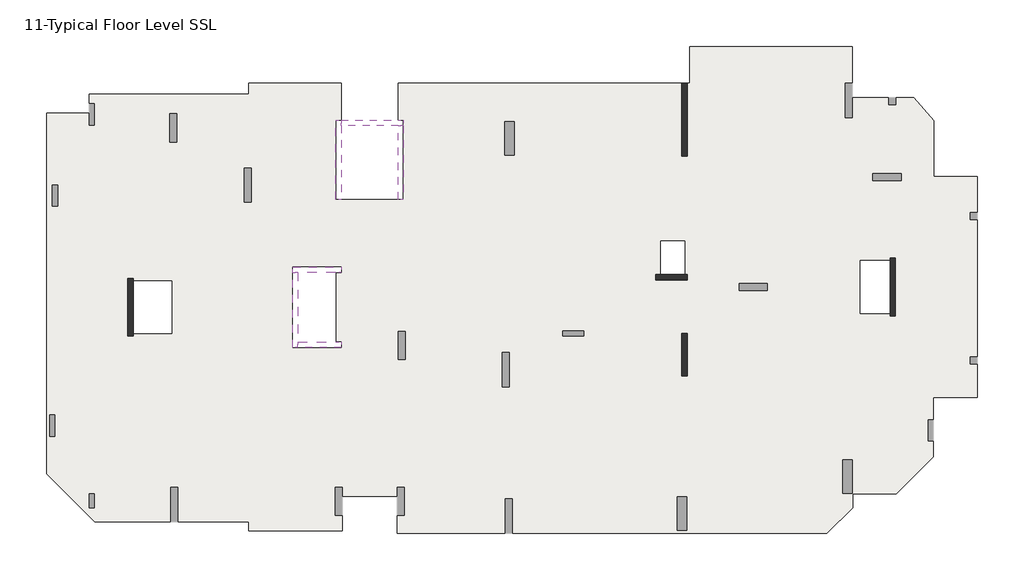
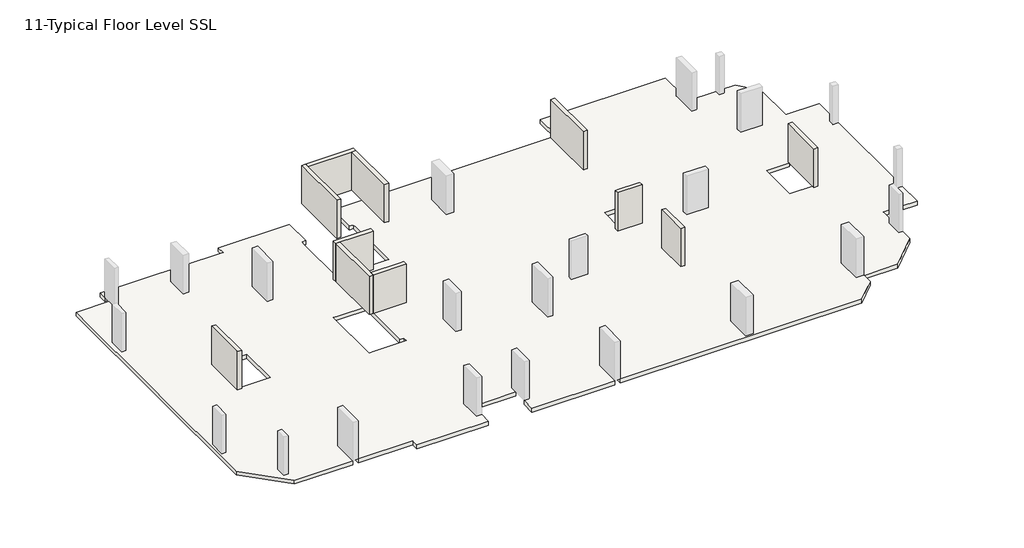
# One storey, part 1 of 2: 11 walls, 1 slab.
"""IFC4 building model written with IfcOpenShell, lengths in millimetres."""

from ifc_helpers import new_model, si_unit, origin, place, context, project, spatial, faceted_brep, element, save

model = new_model("IFC4")

# Units and contexts
model_context = context("Model", 3, world=origin())
ifc_project = project(units=[si_unit("LENGTHUNIT", "METRE", prefix="MILLI")], contexts=[model_context])

# Site, building, storey
site = spatial("IfcSite", under=ifc_project)
building = spatial("IfcBuilding", under=site)
storey = spatial("IfcBuildingStorey", under=building, Name="11-Typical Floor Level SSL", Elevation=27000.0)

# Slab
placement = place(None, origin())
element("IfcSlab", 1, ObjectType="Generic 300mm", at=placement, inside=storey, context=model_context, shape_type="Brep", body=[
    faceted_brep([(36192.0021644, 24072.000519, 26700.0), (36192.0021644, 26172.000519, 26700.0), (45446.0007483, 26172.000519, 26700.0), (45446.0007483, 24087.0, 26700.0), (45046.0007483, 24087.0, 26700.0), (45046.0007483, 22137.0, 26700.0), (45446.0007483, 22137.0, 26700.0), (45446.0007483, 23252.0000315, 26700.0), (47498.6337868, 23252.0000315, 26700.0), (47498.6337868, 22852.0, 26700.0), (47898.6337868, 22852.0, 26700.0), (47898.6337868, 23252.0000315, 26700.0), (48936.764334, 23252.0000315, 26700.0), (50076.0016214, 21956.8283806, 26700.0), (50076.0016214, 18780.0084406, 26700.0), (52549.9999998, 18780.0084406, 26700.0), (52549.9999998, 16712.0, 26700.0), (52149.9999998, 16712.0, 26700.0), (52149.9999998, 16312.0, 26700.0), (52549.9999998, 16312.0, 26700.0), (52549.9999998, 8504.0039609, 26700.0), (52149.9999998, 8504.0039609, 26700.0), (52149.9999998, 8104.0039609, 26700.0), (52549.9999998, 8104.0039609, 26700.0), (52549.9999998, 6204.0084406, 26700.0), (50046.0009271, 6204.0084406, 26700.0), (50046.0009271, 4931.9999929, 26700.0), (49746.0009271, 4931.9999929, 26700.0), (49746.0009271, 3731.9999929, 26700.0), (50046.0009271, 3731.9999929, 26700.0), (50046.0009271, 2810.5958657, 26700.0), (47943.4055804, 708.000519, 26700.0), (45456.0017287, 708.000519, 26700.0), (45456.0017287, -61.7051085, 26700.0), (43990.7023722, -1527.004465, 26700.0), (26113.9999998, -1527.004465, 26700.0), (26113.9999998, 422.995535, 26700.0), (25713.9999998, 422.995535, 26700.0), (25713.9999998, -1527.004465, 26700.0), (19569.9997488, -1527.004465, 26700.0), (19569.9997488, -512.0044652, 26700.0), (19969.9997488, -512.0044652, 26700.0), (19969.9997488, 1087.9955348, 26700.0), (19569.9997488, 1087.9955348, 26700.0), (19569.9997488, 564.000519, 26700.0), (16429.9999981, 564.000519, 26700.0), (16429.9999981, 1088.0, 26700.0), (16029.9999981, 1088.0, 26700.0), (16029.9999981, -512.0, 26700.0), (16429.9999981, -512.0, 26700.0), (16429.9999981, -1391.999481, 26700.0), (11136.0000923, -1391.999481, 26700.0), (11136.0000923, -866.9999847, 26700.0), (7082.0000416, -866.9999847, 26700.0), (7082.0000416, 1083.0000153, 26700.0), (6682.0000416, 1083.0000153, 26700.0), (6682.0000416, -866.9999847, 26700.0), (2364.4419097, -866.9999847, 26700.0), (-372.0, 1869.441925, 26700.0), (-372.0, 22380.0004589, 26700.0), (2052.0, 22380.0004589, 26700.0), (2052.0, 21708.0000656, 26700.0), (2352.0, 21708.0000656, 26700.0), (2352.0, 22908.0000656, 26700.0), (2052.0, 22908.0000656, 26700.0), (2052.0, 23472.000519, 26700.0), (11136.0000923, 23472.000519, 26700.0), (11136.0000923, 24072.000519, 26700.0), (16380.0000168, 24072.000519, 26700.0), (16380.0000168, 21972.0, 26700.0), (16079.9999997, 21972.0, 26700.0), (16079.9999997, 21672.0, 26700.0), (16079.9999997, 17468.0, 26700.0), (16379.9999997, 17468.0, 26700.0), (19619.9999997, 17468.0, 26700.0), (19919.9999997, 17468.0, 26700.0), (19919.9999997, 21672.0, 26700.0), (19919.9999997, 21972.0, 26700.0), (19619.9997365, 21972.0, 26700.0), (19619.9997365, 24072.000519, 26700.0), (35747.9999998, 24072.000519, 26700.0), (35747.9999998, 19932.0, 26700.0), (36047.9999998, 19932.0, 26700.0), (36047.9999998, 24072.000519, 26700.0), (16079.9999907, 9359.999998, 26700.0), (16079.9999907, 13320.0000002, 26700.0), (16380.0000168, 13320.0000002, 26700.0), (16380.0000168, 13620.0000002, 26700.0), (13919.9999907, 13620.0000002, 26700.0), (13619.9999907, 13620.0000002, 26700.0), (13619.9999907, 13320.0000002, 26700.0), (13619.9999907, 9359.999998, 26700.0), (13619.9999907, 9059.999998, 26700.0), (13919.9999907, 9059.999998, 26700.0), (16380.0000168, 9059.999998, 26700.0), (16380.0000168, 9359.999998, 26700.0), (4548.0000034, 9840.0000003, 26700.0), (6743.9999995, 9840.0000003, 26700.0), (6743.9999995, 12840.0000003, 26700.0), (4548.0000034, 12840.0000003, 26700.0), (4548.0000025, 12984.0000001, 26700.0), (4248.0000025, 12984.0000001, 26700.0), (4248.0000025, 9696.0, 26700.0), (4548.0000025, 9696.0, 26700.0), (47580.0014798, 13992.0079177, 26700.0), (45900.001729, 13992.0079177, 26700.0), (45900.001729, 10992.0079181, 26700.0), (47580.0014798, 10992.0079181, 26700.0), (47580.0014811, 10848.0079202, 26700.0), (47880.0014811, 10848.0079202, 26700.0), (47880.0014811, 14136.0000002, 26700.0), (47580.0014811, 14136.0000002, 26700.0), (35904.002157, 15108.0000083, 26700.0), (34548.0015145, 15108.0000083, 26700.0), (34548.0015145, 13199.9999992, 26700.0), (34248.0015201, 13199.9999992, 26700.0), (34248.0015201, 12899.9999992, 26700.0), (36048.0015201, 12899.9999992, 26700.0), (36048.0015201, 13199.9999992, 26700.0), (35904.002157, 13199.9999992, 26700.0), (257.9999999, 17088.0, 26700.0), (257.9999999, 18288.0, 26700.0), (-42.0000001, 18288.0, 26700.0), (-42.0000001, 17088.0, 26700.0), (108.001803, 4001.9999858, 26700.0), (108.001803, 5201.9999858, 26700.0), (-191.998197, 5201.9999858, 26700.0), (-191.998197, 4001.9999858, 26700.0), (30175.9999998, 9996.0000019, 26700.0), (28975.9999998, 9996.0000019, 26700.0), (28975.9999998, 9696.0000019, 26700.0), (30175.9999998, 9696.0000019, 26700.0), (7021.9999999, 20740.0000078, 26700.0), (7021.9999999, 22340.0000078, 26700.0), (6621.9999999, 22340.0000078, 26700.0), (6621.9999999, 20740.0000078, 26700.0), (48205.9993605, 18950.0, 26700.0), (46605.9993605, 18950.0, 26700.0), (46605.9993605, 18550.0, 26700.0), (48205.9993605, 18550.0, 26700.0), (20030.000009, 8355.9999979, 26700.0), (20030.000009, 9955.9999979, 26700.0), (19630.000009, 9955.9999979, 26700.0), (19630.000009, 8355.9999979, 26700.0), (11270.0000427, 17312.9999996, 26700.0), (11270.0000427, 19262.9999996, 26700.0), (10870.0000427, 19262.9999996, 26700.0), (10870.0000427, 17312.9999996, 26700.0), (40598.0014887, 12692.0079212, 26700.0), (38998.0014887, 12692.0079212, 26700.0), (38998.0014887, 12292.0079212, 26700.0), (40598.0014887, 12292.0079212, 26700.0), (2352.0, -72.0, 26700.0), (2352.0, 728.0, 26700.0), (2052.0, 728.0, 26700.0), (2052.0, -72.0, 26700.0), (25934.0000455, 6801.0001824, 26700.0), (25934.0000455, 8751.0001824, 26700.0), (25534.0000455, 8751.0001824, 26700.0), (25534.0000455, 6801.0001824, 26700.0), (36035.9999998, -1351.9992017, 26700.0), (36035.9999998, 548.0007983, 26700.0), (35485.9999998, 548.0007983, 26700.0), (35485.9999998, -1351.9992017, 26700.0), (45443.9999998, 748.0, 26700.0), (45443.9999998, 2648.0, 26700.0), (44893.9999998, 2648.0, 26700.0), (44893.9999998, 748.0, 26700.0), (26218.9999998, 20000.0, 26700.0), (26218.9999998, 21900.0, 26700.0), (25668.9999998, 21900.0, 26700.0), (25668.9999998, 20000.0, 26700.0), (35748.0054035, 9840.0000002, 26700.0), (35748.0054035, 7428.0000762, 26700.0), (36048.0054035, 7428.0000762, 26700.0), (36048.0054035, 9840.0000002, 26700.0), (36192.0021644, 26172.000519, 27000.0), (36192.0021644, 24072.000519, 27000.0), (36047.9999998, 24072.000519, 27000.0), (36047.9999998, 19932.0, 27000.0), (35747.9999998, 19932.0, 27000.0), (35747.9999998, 24072.000519, 27000.0), (19619.9997365, 24072.000519, 27000.0), (19619.9997365, 21972.0, 27000.0), (19919.9999997, 21972.0, 27000.0), (19919.9999997, 21672.0, 27000.0), (19919.9999997, 17468.0, 27000.0), (19619.9999997, 17468.0, 27000.0), (16379.9999997, 17468.0, 27000.0), (16079.9999997, 17468.0, 27000.0), (16079.9999997, 21672.0, 27000.0), (16079.9999997, 21972.0, 27000.0), (16380.0000168, 21972.0, 27000.0), (16380.0000168, 24072.000519, 27000.0), (11136.0000923, 24072.000519, 27000.0), (11136.0000923, 23472.000519, 27000.0), (2052.0, 23472.000519, 27000.0), (2052.0, 22908.0000656, 27000.0), (2352.0, 22908.0000656, 27000.0), (2352.0, 21708.0000656, 27000.0), (2052.0, 21708.0000656, 27000.0), (2052.0, 22380.0004589, 27000.0), (-372.0, 22380.0004589, 27000.0), (-372.0, 1869.441925, 27000.0), (2364.4419097, -866.9999847, 27000.0), (6682.0000416, -866.9999847, 27000.0), (6682.0000416, 1083.0000153, 27000.0), (7082.0000416, 1083.0000153, 27000.0), (7082.0000416, -866.9999847, 27000.0), (11136.0000923, -866.9999847, 27000.0), (11136.0000923, -1391.999481, 27000.0), (16429.9999981, -1391.999481, 27000.0), (16429.9999981, -512.0, 27000.0), (16029.9999981, -512.0, 27000.0), (16029.9999981, 1088.0, 27000.0), (16429.9999981, 1088.0, 27000.0), (16429.9999981, 564.000519, 27000.0), (19569.9997488, 564.000519, 27000.0), (19569.9997488, 1087.9955348, 27000.0), (19969.9997488, 1087.9955348, 27000.0), (19969.9997488, -512.0044652, 27000.0), (19569.9997488, -512.0044652, 27000.0), (19569.9997488, -1527.004465, 27000.0), (25713.9999998, -1527.004465, 27000.0), (25713.9999998, 422.995535, 27000.0), (26113.9999998, 422.995535, 27000.0), (26113.9999998, -1527.004465, 27000.0), (43990.7023722, -1527.004465, 27000.0), (45456.0017287, -61.7051085, 27000.0), (45456.0017287, 708.000519, 27000.0), (47943.4055804, 708.000519, 27000.0), (50046.0009271, 2810.5958657, 27000.0), (50046.0009271, 3731.9999929, 27000.0), (49746.0009271, 3731.9999929, 27000.0), (49746.0009271, 4931.9999929, 27000.0), (50046.0009271, 4931.9999929, 27000.0), (50046.0009271, 6204.0084406, 27000.0), (52549.9999998, 6204.0084406, 27000.0), (52549.9999998, 8104.0039609, 27000.0), (52149.9999998, 8104.0039609, 27000.0), (52149.9999998, 8504.0039609, 27000.0), (52549.9999998, 8504.0039609, 27000.0), (52549.9999998, 16312.0, 27000.0), (52149.9999998, 16312.0, 27000.0), (52149.9999998, 16712.0, 27000.0), (52549.9999998, 16712.0, 27000.0), (52549.9999998, 18780.0084406, 27000.0), (50076.0016214, 18780.0084406, 27000.0), (50076.0016214, 21956.8283806, 27000.0), (48936.764334, 23252.0000315, 27000.0), (47898.6337868, 23252.0000315, 27000.0), (47898.6337868, 22852.0, 27000.0), (47498.6337868, 22852.0, 27000.0), (47498.6337868, 23252.0000315, 27000.0), (45446.0006898, 23252.0000315, 27000.0), (45446.0007483, 22137.0, 27000.0), (45046.0007483, 22137.0, 27000.0), (45046.0007483, 24087.0, 27000.0), (45446.0007483, 24087.0, 27000.0), (45446.0007483, 26172.000519, 27000.0), (16079.9999907, 13320.0000002, 27000.0), (16079.9999907, 9359.999998, 27000.0), (16380.0000168, 9359.999998, 27000.0), (16380.0000168, 9059.999998, 27000.0), (13919.9999907, 9059.999998, 27000.0), (13619.9999907, 9059.999998, 27000.0), (13619.9999907, 9359.999998, 27000.0), (13619.9999907, 13320.0000002, 27000.0), (13619.9999907, 13620.0000002, 27000.0), (13919.9999907, 13620.0000002, 27000.0), (16380.0000168, 13620.0000002, 27000.0), (16380.0000168, 13320.0000002, 27000.0), (6743.9999995, 9840.0000003, 27000.0), (4548.0000034, 9840.0000003, 27000.0), (4548.0000025, 9696.0, 27000.0), (4248.0000025, 9696.0, 27000.0), (4248.0000025, 12984.0000001, 27000.0), (4548.0000025, 12984.0000001, 27000.0), (4548.0000025, 12840.0000003, 27000.0), (6743.9999995, 12840.0000003, 27000.0), (45900.001729, 13992.0079177, 27000.0), (47580.0014798, 13992.0079177, 27000.0), (47580.0014811, 14136.0000002, 27000.0), (47880.0014811, 14136.0000002, 27000.0), (47880.0014811, 10848.0079202, 27000.0), (47580.0014811, 10848.0079202, 27000.0), (47580.0014811, 10992.0079181, 27000.0), (45900.001729, 10992.0079181, 27000.0), (34548.0015145, 15108.0000083, 27000.0), (35904.002157, 15108.0000083, 27000.0), (35904.002157, 13199.9999992, 27000.0), (36048.0015201, 13199.9999992, 27000.0), (36048.0015201, 12899.9999992, 27000.0), (34248.0015201, 12899.9999992, 27000.0), (34248.0015201, 13199.9999992, 27000.0), (34548.0015145, 13199.9999992, 27000.0), (257.9999999, 18288.0, 27000.0), (257.9999999, 17088.0, 27000.0), (-42.0000001, 17088.0, 27000.0), (-42.0000001, 18288.0, 27000.0), (108.001803, 5201.9999858, 27000.0), (108.001803, 4001.9999858, 27000.0), (-191.998197, 4001.9999858, 27000.0), (-191.998197, 5201.9999858, 27000.0), (28975.9999998, 9996.0000019, 27000.0), (30175.9999998, 9996.0000019, 27000.0), (30175.9999998, 9696.0000019, 27000.0), (28975.9999998, 9696.0000019, 27000.0), (7021.9999999, 22340.0000078, 27000.0), (7021.9999999, 20740.0000078, 27000.0), (6621.9999999, 20740.0000078, 27000.0), (6621.9999999, 22340.0000078, 27000.0), (46605.9993605, 18950.0, 27000.0), (48205.9993605, 18950.0, 27000.0), (48205.9993605, 18550.0, 27000.0), (46605.9993605, 18550.0, 27000.0), (20030.000009, 9955.9999979, 27000.0), (20030.000009, 8355.9999979, 27000.0), (19630.000009, 8355.9999979, 27000.0), (19630.000009, 9955.9999979, 27000.0), (11270.0000427, 19262.9999996, 27000.0), (11270.0000427, 17312.9999996, 27000.0), (10870.0000427, 17312.9999996, 27000.0), (10870.0000427, 19262.9999996, 27000.0), (38998.0014887, 12692.0079212, 27000.0), (40598.0014887, 12692.0079212, 27000.0), (40598.0014887, 12292.0079212, 27000.0), (38998.0014887, 12292.0079212, 27000.0), (2352.0, 728.0, 27000.0), (2352.0, -72.0, 27000.0), (2052.0, -72.0, 27000.0), (2052.0, 728.0, 27000.0), (25934.0000455, 8751.0001824, 27000.0), (25934.0000455, 6801.0001824, 27000.0), (25534.0000455, 6801.0001824, 27000.0), (25534.0000455, 8751.0001824, 27000.0), (36035.9999998, 548.0007983, 27000.0), (36035.9999998, -1351.9992017, 27000.0), (35485.9999998, -1351.9992017, 27000.0), (35485.9999998, 548.0007983, 27000.0), (45443.9999998, 2648.0, 27000.0), (45443.9999998, 748.0, 27000.0), (44893.9999998, 748.0, 27000.0), (44893.9999998, 2648.0, 27000.0), (26218.9999998, 21900.0, 27000.0), (26218.9999998, 20000.0, 27000.0), (25668.9999998, 20000.0, 27000.0), (25668.9999998, 21900.0, 27000.0), (35748.0054035, 7428.0000762, 27000.0), (35748.0054035, 9840.0000002, 27000.0), (36048.0054035, 9840.0000002, 27000.0), (36048.0054035, 7428.0000762, 27000.0)], [[[0, 1, 2, 3, 4, 5, 6, 7, 8, 9, 10, 11, 12, 13, 14, 15, 16, 17, 18, 19, 20, 21, 22, 23, 24, 25, 26, 27, 28, 29, 30, 31, 32, 33, 34, 35, 36, 37, 38, 39, 40, 41, 42, 43, 44, 45, 46, 47, 48, 49, 50, 51, 52, 53, 54, 55, 56, 57, 58, 59, 60, 61, 62, 63, 64, 65, 66, 67, 68, 69, 70, 71, 72, 73, 74, 75, 76, 77, 78, 79, 80, 81, 82, 83], [84, 85, 86, 87, 88, 89, 90, 91, 92, 93, 94, 95], [96, 97, 98, 99, 100, 101, 102, 103], [104, 105, 106, 107, 108, 109, 110, 111], [112, 113, 114, 115, 116, 117, 118, 119], [120, 121, 122, 123], [124, 125, 126, 127], [128, 129, 130, 131], [132, 133, 134, 135], [136, 137, 138, 139], [140, 141, 142, 143], [144, 145, 146, 147], [148, 149, 150, 151], [152, 153, 154, 155], [156, 157, 158, 159], [160, 161, 162, 163], [164, 165, 166, 167], [168, 169, 170, 171], [172, 173, 174, 175]], [[176, 177, 178, 179, 180, 181, 182, 183, 184, 185, 186, 187, 188, 189, 190, 191, 192, 193, 194, 195, 196, 197, 198, 199, 200, 201, 202, 203, 204, 205, 206, 207, 208, 209, 210, 211, 212, 213, 214, 215, 216, 217, 218, 219, 220, 221, 222, 223, 224, 225, 226, 227, 228, 229, 230, 231, 232, 233, 234, 235, 236, 237, 238, 239, 240, 241, 242, 243, 244, 245, 246, 247, 248, 249, 250, 251, 252, 253, 254, 255, 256, 257, 258, 259], [260, 261, 262, 263, 264, 265, 266, 267, 268, 269, 270, 271], [272, 273, 274, 275, 276, 277, 278, 279], [280, 281, 282, 283, 284, 285, 286, 287], [288, 289, 290, 291, 292, 293, 294, 295], [296, 297, 298, 299], [300, 301, 302, 303], [304, 305, 306, 307], [308, 309, 310, 311], [312, 313, 314, 315], [316, 317, 318, 319], [320, 321, 322, 323], [324, 325, 326, 327], [328, 329, 330, 331], [332, 333, 334, 335], [336, 337, 338, 339], [340, 341, 342, 343], [344, 345, 346, 347], [348, 349, 350, 351]], [[68, 193, 192, 69]], [[182, 79, 78, 183]], [[79, 182, 181, 80]], [[177, 0, 83, 178]], [[1, 0, 177, 176]], [[2, 1, 176, 259]], [[3, 2, 259, 258]], [[249, 12, 11, 250]], [[7, 254, 253, 8]], [[13, 12, 249, 248]], [[14, 13, 248, 247]], [[15, 14, 247, 246]], [[15, 246, 245, 16]], [[237, 24, 23, 238]], [[19, 242, 241, 20]], [[25, 24, 237, 236]], [[25, 236, 235, 26]], [[231, 30, 29, 232]], [[32, 31, 230, 229]], [[33, 32, 229, 228]], [[34, 33, 228, 227]], [[34, 227, 226, 35]], [[222, 39, 38, 223]], [[39, 222, 221, 40]], [[45, 44, 217, 216]], [[211, 50, 49, 212]], [[51, 50, 211, 210]], [[52, 51, 210, 209]], [[52, 209, 208, 53]], [[204, 57, 56, 205]], [[58, 57, 204, 203]], [[59, 58, 203, 202]], [[60, 59, 202, 201]], [[196, 65, 64, 197]], [[66, 65, 196, 195]], [[67, 66, 195, 194]], [[68, 67, 194, 193]], [[31, 30, 231, 230]], [[85, 84, 261, 260]], [[72, 189, 188, 187, 186, 75, 74, 73]], [[272, 97, 96, 273]], [[97, 272, 279, 98]], [[98, 279, 278, 99]], [[280, 105, 104, 281]], [[105, 280, 287, 106]], [[106, 287, 286, 107]], [[112, 289, 288, 113]], [[113, 288, 295, 114]], [[289, 112, 119, 290]], [[62, 199, 198, 63]], [[199, 62, 61, 200]], [[200, 61, 60, 201]], [[63, 198, 197, 64]], [[120, 297, 296, 121]], [[297, 120, 123, 298]], [[298, 123, 122, 299]], [[299, 122, 121, 296]], [[124, 301, 300, 125]], [[301, 124, 127, 302]], [[302, 127, 126, 303]], [[303, 126, 125, 300]], [[28, 233, 232, 29]], [[233, 28, 27, 234]], [[234, 27, 26, 235]], [[128, 305, 304, 129]], [[305, 128, 131, 306]], [[306, 131, 130, 307]], [[307, 130, 129, 304]], [[132, 309, 308, 133]], [[309, 132, 135, 310]], [[310, 135, 134, 311]], [[311, 134, 133, 308]], [[41, 220, 219, 42]], [[220, 41, 40, 221]], [[43, 218, 217, 44]], [[218, 43, 42, 219]], [[136, 313, 312, 137]], [[313, 136, 139, 314]], [[314, 139, 138, 315]], [[315, 138, 137, 312]], [[140, 317, 316, 141]], [[317, 140, 143, 318]], [[318, 143, 142, 319]], [[319, 142, 141, 316]], [[215, 46, 45, 216]], [[48, 213, 212, 49]], [[213, 48, 47, 214]], [[214, 47, 46, 215]], [[144, 321, 320, 145]], [[321, 144, 147, 322]], [[322, 147, 146, 323]], [[323, 146, 145, 320]], [[207, 54, 53, 208]], [[55, 206, 205, 56]], [[206, 55, 54, 207]], [[225, 36, 35, 226]], [[37, 224, 223, 38]], [[224, 37, 36, 225]], [[6, 255, 254, 7]], [[255, 6, 5, 256]], [[256, 5, 4, 257]], [[257, 4, 3, 258]], [[148, 325, 324, 149]], [[325, 148, 151, 326]], [[326, 151, 150, 327]], [[327, 150, 149, 324]], [[152, 329, 328, 153]], [[329, 152, 155, 330]], [[330, 155, 154, 331]], [[331, 154, 153, 328]], [[156, 333, 332, 157]], [[333, 156, 159, 334]], [[334, 159, 158, 335]], [[335, 158, 157, 332]], [[160, 337, 336, 161]], [[337, 160, 163, 338]], [[338, 163, 162, 339]], [[339, 162, 161, 336]], [[164, 341, 340, 165]], [[341, 164, 167, 342]], [[342, 167, 166, 343]], [[343, 166, 165, 340]], [[168, 345, 344, 169]], [[345, 168, 171, 346]], [[346, 171, 170, 347]], [[347, 170, 169, 344]], [[70, 191, 190, 189, 72, 71]], [[191, 70, 69, 192]], [[77, 184, 183, 78]], [[184, 77, 76, 75, 186, 185]], [[271, 86, 85, 260]], [[87, 270, 269, 268, 89, 88]], [[86, 271, 270, 87]], [[89, 268, 267, 266, 265, 92, 91, 90]], [[92, 265, 264, 263, 94, 93]], [[95, 262, 261, 84]], [[262, 95, 94, 263]], [[277, 100, 99, 278]], [[103, 274, 273, 96]], [[101, 276, 275, 102]], [[100, 277, 276, 101]], [[274, 103, 102, 275]], [[116, 293, 292, 117]], [[118, 291, 290, 119]], [[294, 115, 114, 295]], [[117, 292, 291, 118]], [[293, 116, 115, 294]], [[172, 349, 348, 173]], [[174, 351, 350, 175]], [[173, 348, 351, 174]], [[349, 172, 175, 350]], [[285, 108, 107, 286]], [[111, 282, 281, 104]], [[109, 284, 283, 110]], [[108, 285, 284, 109]], [[282, 111, 110, 283]], [[82, 179, 178, 83]], [[180, 81, 80, 181]], [[179, 82, 81, 180]], [[18, 243, 242, 19]], [[243, 18, 17, 244]], [[244, 17, 16, 245]], [[10, 251, 250, 11]], [[251, 10, 9, 252]], [[252, 9, 8, 253]], [[22, 239, 238, 23]], [[239, 22, 21, 240]], [[240, 21, 20, 241]]]),
])

# Walls
element("IfcWall", 2, ObjectType="Shear Walls 300mm", at=placement, inside=storey, context=model_context, shape_type="Brep", body=[
    faceted_brep([(4548.0000025, 9696.0, 27000.0), (4548.0000025, 12984.0000001, 27000.0), (4548.0000025, 12984.0000001, 29700.0), (4548.0000025, 12984.0000001, 30000.0), (4548.0000025, 12840.0000003, 30000.0), (4548.0000025, 9840.0000003, 30000.0), (4548.0000025, 9696.0, 30000.0), (4548.0000025, 9696.0, 29700.0), (4248.0000025, 9696.0, 27000.0), (4248.0000025, 9696.0, 29700.0), (4248.0000025, 9696.0, 30000.0), (4248.0000025, 12984.0000001, 30000.0), (4248.0000025, 12984.0000001, 29700.0), (4248.0000025, 12984.0000001, 27000.0)], [[[0, 1, 2, 3, 4, 5, 6, 7]], [[8, 9, 10, 11, 12, 13]], [[1, 0, 8, 13]], [[3, 2, 1, 13, 12, 11]], [[6, 5, 4, 3, 11, 10]], [[0, 7, 6, 10, 9, 8]]]),
])
element("IfcWall", 3, ObjectType="Shear Walls 300mm", at=placement, inside=storey, context=model_context, shape_type="Brep", body=[
    faceted_brep([(34248.0015201, 12899.9999992, 27000.0), (36048.0015201, 12899.9999992, 27000.0), (36048.0015201, 12899.9999992, 29700.0), (36048.0015201, 12899.9999992, 30000.0), (34248.0015201, 12899.9999992, 30000.0), (34248.0015201, 12899.9999992, 29700.0), (34248.0015201, 13199.9999992, 27000.0), (34248.0015201, 13199.9999992, 29700.0), (34248.0015201, 13199.9999992, 30000.0), (34548.0015145, 13199.9999992, 30000.0), (35904.002157, 13199.9999992, 30000.0), (36048.0015201, 13199.9999992, 30000.0), (36048.0015201, 13199.9999992, 29700.0), (36048.0015201, 13199.9999992, 27000.0)], [[[0, 1, 2, 3, 4, 5]], [[6, 7, 8, 9, 10, 11, 12, 13]], [[1, 0, 6, 13]], [[3, 2, 1, 13, 12, 11]], [[4, 3, 11, 10, 9, 8]], [[0, 5, 4, 8, 7, 6]]]),
])
element("IfcWall", 4, ObjectType="Shear Walls 300mm", at=placement, inside=storey, context=model_context, shape_type="Brep", body=[
    faceted_brep([(35748.0054035, 9840.0000002, 27000.0), (35748.0054035, 7428.0000762, 27000.0), (35748.0054035, 7428.0000762, 29700.0), (35748.0054035, 7428.0000762, 30000.0), (35748.0054035, 9840.0000002, 30000.0), (35748.0054035, 9840.0000002, 29700.0), (36048.0054035, 9840.0000002, 27000.0), (36048.0054035, 9840.0000002, 29700.0), (36048.0054035, 9840.0000002, 30000.0), (36048.0054035, 7428.0000762, 30000.0), (36048.0054035, 7428.0000762, 29700.0), (36048.0054035, 7428.0000762, 27000.0)], [[[0, 1, 2, 3, 4, 5]], [[6, 7, 8, 9, 10, 11]], [[1, 0, 6, 11]], [[3, 2, 1, 11, 10, 9]], [[4, 3, 9, 8]], [[0, 5, 4, 8, 7, 6]]]),
])
element("IfcWall", 5, ObjectType="Shear Walls 300mm", at=placement, inside=storey, context=model_context, shape_type="Brep", body=[
    faceted_brep([(47580.0014811, 14136.0000002, 27000.0), (47580.0014811, 10848.0079202, 27000.0), (47580.0014811, 10848.0079202, 29700.0), (47580.0014811, 10848.0079202, 30000.0), (47580.0014811, 10992.0079181, 30000.0), (47580.0014811, 13992.0079177, 30000.0), (47580.0014811, 14136.0000002, 30000.0), (47580.0014811, 14136.0000002, 29700.0), (47880.0014811, 14136.0000002, 27000.0), (47880.0014811, 14136.0000002, 29700.0), (47880.0014811, 14136.0000002, 30000.0), (47880.0014811, 10848.0079202, 30000.0), (47880.0014811, 10848.0079202, 29700.0), (47880.0014811, 10848.0079202, 27000.0)], [[[0, 1, 2, 3, 4, 5, 6, 7]], [[8, 9, 10, 11, 12, 13]], [[1, 0, 8, 13]], [[3, 2, 1, 13, 12, 11]], [[6, 5, 4, 3, 11, 10]], [[0, 7, 6, 10, 9, 8]]]),
])
element("IfcWall", 6, ObjectType="Shear Walls 300mm", at=placement, inside=storey, context=model_context, shape_type="Brep", body=[
    faceted_brep([(36047.9999998, 19932.0, 27000.0), (36047.9999998, 24072.0078999, 27000.0), (36047.9999998, 24072.0078999, 30000.0), (36047.9999998, 19932.0, 30000.0), (36047.9999998, 19932.0, 29700.0), (35747.9999998, 19932.0, 27000.0), (35747.9999998, 19932.0, 29700.0), (35747.9999998, 19932.0, 30000.0), (35747.9999998, 24072.0078999, 30000.0), (35747.9999998, 24072.0078999, 27000.0)], [[[0, 1, 2, 3, 4]], [[5, 6, 7, 8, 9]], [[1, 0, 5, 9]], [[2, 1, 9, 8]], [[3, 2, 8, 7]], [[0, 4, 3, 7, 6, 5]]]),
])
element("IfcWall", 7, ObjectType="Shear Walls 300mm", at=placement, inside=storey, context=model_context, shape_type="Brep", body=[
    faceted_brep([(16379.9999997, 21972.0, 33000.0), (16379.9999997, 21672.0, 33000.0), (16379.9999997, 17468.0, 33000.0), (16379.9999997, 17468.0, 30000.0), (16379.9999997, 21672.0, 30000.0), (16379.9999997, 21972.0, 30000.0), (16079.9999997, 17468.0, 33000.0), (16079.9999997, 21972.0, 33000.0), (16079.9999997, 21972.0, 32700.0), (16079.9999997, 21972.0, 30000.0), (16079.9999997, 17468.0, 30000.0), (16079.9999997, 17468.0, 32700.0)], [[[0, 1, 2, 3, 4, 5]], [[6, 7, 8, 9, 10, 11]], [[2, 1, 0, 7, 6]], [[2, 6, 11, 10, 3]], [[3, 10, 9, 5, 4]], [[0, 5, 9, 8, 7]]]),
])
element("IfcWall", 8, ObjectType="Shear Walls 300mm", at=placement, inside=storey, context=model_context, shape_type="Brep", body=[
    faceted_brep([(16379.9999997, 21972.0, 33000.0), (19619.9997365, 21972.0, 33000.0), (19919.9999997, 21972.0, 33000.0), (19919.9999997, 21972.0, 32700.0), (19919.9999997, 21972.0, 30000.0), (16379.9999997, 21972.0, 30000.0), (19919.9999997, 21672.0, 33000.0), (19619.9999997, 21672.0, 33000.0), (16379.9999997, 21672.0, 33000.0), (16379.9999997, 21672.0, 30000.0), (19619.9999997, 21672.0, 30000.0), (19919.9999997, 21672.0, 30000.0)], [[[0, 1, 2, 3, 4, 5]], [[6, 7, 8, 9, 10, 11]], [[2, 1, 0, 8, 7, 6]], [[8, 0, 5, 9]], [[9, 5, 4, 11, 10]], [[4, 3, 2, 6, 11]]]),
])
element("IfcWall", 9, ObjectType="Shear Walls 300mm", at=placement, inside=storey, context=model_context, shape_type="Brep", body=[
    faceted_brep([(19919.9999997, 21672.0, 33000.0), (19919.9999997, 17468.0, 33000.0), (19919.9999997, 17468.0, 32700.0), (19919.9999997, 17468.0, 30000.0), (19919.9999997, 21672.0, 30000.0), (19619.9999997, 17468.0, 33000.0), (19619.9999997, 21672.0, 33000.0), (19619.9999997, 21672.0, 30000.0), (19619.9999997, 17468.0, 30000.0)], [[[0, 1, 2, 3, 4]], [[5, 6, 7, 8]], [[1, 0, 6, 5]], [[1, 5, 8, 3, 2]], [[6, 0, 4, 7]], [[4, 3, 8, 7]]]),
])
element("IfcWall", 10, ObjectType="Shear Walls 300mm", at=placement, inside=storey, context=model_context, shape_type="Brep", body=[
    faceted_brep([(16380.0000168, 13320.0000002, 33000.0), (16079.9999907, 13320.0000002, 33000.0), (13919.9999907, 13320.0000002, 33000.0), (13619.9999907, 13320.0000002, 33000.0), (13619.9999907, 13320.0000002, 30000.0), (13919.9999907, 13320.0000002, 30000.0), (16380.0000168, 13320.0000002, 30000.0), (16380.0000168, 13320.0000002, 32700.0), (13619.9999907, 13620.0000002, 33000.0), (16380.0000168, 13620.0000002, 33000.0), (16380.0000168, 13620.0000002, 32700.0), (16380.0000168, 13620.0000002, 30000.0), (13619.9999907, 13620.0000002, 30000.0), (13619.9999907, 13620.0000002, 32700.0)], [[[0, 1, 2, 3, 4, 5, 6, 7]], [[8, 9, 10, 11, 12, 13]], [[9, 0, 7, 6, 11, 10]], [[3, 2, 1, 0, 9, 8]], [[11, 6, 5, 4, 12]], [[4, 3, 8, 13, 12]]]),
])
element("IfcWall", 11, ObjectType="Shear Walls 300mm", at=placement, inside=storey, context=model_context, shape_type="Brep", body=[
    faceted_brep([(13919.9999907, 13320.0000002, 33000.0), (13919.9999907, 9359.999998, 33000.0), (13919.9999907, 9059.999998, 33000.0), (13919.9999907, 9059.999998, 30000.0), (13919.9999907, 9359.999998, 30000.0), (13919.9999907, 13320.0000002, 30000.0), (13619.9999907, 9059.999998, 33000.0), (13619.9999907, 13320.0000002, 33000.0), (13619.9999907, 13320.0000002, 30000.0), (13619.9999907, 9059.999998, 30000.0), (13619.9999907, 9059.999998, 32700.0)], [[[0, 1, 2, 3, 4, 5]], [[6, 7, 8, 9, 10]], [[2, 1, 0, 7, 6]], [[7, 0, 5, 8]], [[8, 5, 4, 3, 9]], [[3, 2, 6, 10, 9]]]),
])
element("IfcWall", 12, ObjectType="Shear Walls 300mm", at=placement, inside=storey, context=model_context, shape_type="Brep", body=[
    faceted_brep([(13919.9999907, 9359.999998, 33000.0), (16079.9999907, 9359.999998, 33000.0), (16380.0000168, 9359.999998, 33000.0), (16380.0000168, 9359.999998, 32700.0), (16380.0000168, 9359.999998, 30000.0), (13919.9999907, 9359.999998, 30000.0), (16380.0000168, 9059.999998, 33000.0), (13919.9999907, 9059.999998, 33000.0), (13919.9999907, 9059.999998, 30000.0), (16380.0000168, 9059.999998, 30000.0), (16380.0000168, 9059.999998, 32700.0)], [[[0, 1, 2, 3, 4, 5]], [[6, 7, 8, 9, 10]], [[2, 1, 0, 7, 6]], [[2, 6, 10, 9, 4, 3]], [[7, 0, 5, 8]], [[5, 4, 9, 8]]]),
])

save(model, "model.ifc")

# Revit data of these elements
# Type "Generic 300mm"
#   Function = 0
#   Layers, outside or top first: 300 mm "Concrete-RC" (function 1)
# Type "Shear Walls 300mm"
#   Layers, outside or top first: 300 mm "Concrete-RC" (function 1)
# Element 1 (IfcSlab, "Generic 300mm")
#   Height Offset From Level = 0 mm
#   built-in parameter 1001954 = 1
#   Phase Created = New Construction
#   Materials on its faces: "Concrete-RC"
# Elements 2, 3, 4, 5, 6 (IfcWall, "Shear Walls 300mm")
#   Top Offset = 0 mm
#   Base Offset = 0 mm
#   wall height = 3000 mm
#   Phase Created = New Construction
#   Base Constraint = 11-Typical Floor Level SSL
#   Top Constraint = 12-Typical Floor Level SSL
#   Materials on its faces: "Concrete-RC"
# Elements 7, 8, 9, 10, 11, 12 (IfcWall, "Shear Walls 300mm")
#   Top Offset = 0 mm
#   Base Offset = 0 mm
#   wall height = 6000 mm
#   Phase Created = New Construction
#   Base Constraint = 11-Typical Floor Level SSL
#   Top Constraint = 13-Typical Floor Level SSL
#   Materials on its faces: "Concrete-RC"
# Materials
#   "Concrete-RC": class "Concrete", colour RGB 128 128 128, transparency 0, Description = "High strength concrete", Cost = 0
